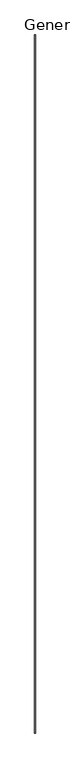
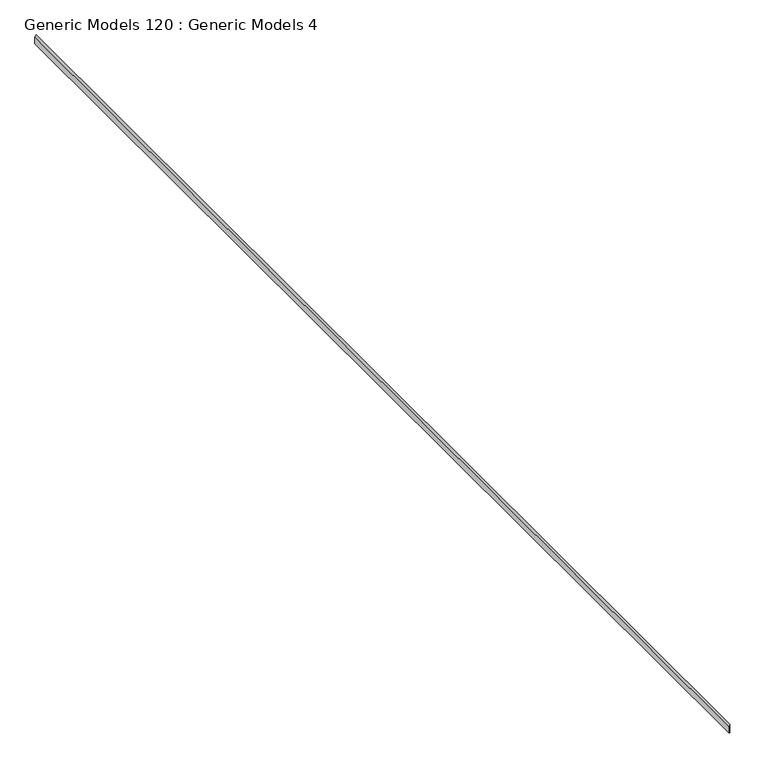
"""IFC4 building model written with IfcOpenShell, lengths in millimetres: proxy geometry, Generic Models 120 : Generic Models 4."""

from ifc_helpers import new_model, si_unit, frame, origin, place, context, project, spatial, polyline, outline, extrude, source, transform, mapped, element, save


def generic_models_120_generic_models_4_1dfd7883(model_context):
    return source(origin(), model_context, "Body", "SweptSolid", [
        extrude(outline(polyline([(126968.835011, 7259.1463704), (126963.120011, 7276.9263704), (127105.8556439, 7276.9263704), (127071.2314334, 7259.1463704), (126968.835011, 7259.1463704)])), frame((0.0, -6864.9230338, 0.0), z_axis=(0.0, 1.0, 0.0), x_axis=(0.0, 0.0, 1.0)), (0.0, 0.0, 1.0), 18643.6),
    ])


if __name__ == "__main__":
    model = new_model("IFC4")
    model_context = context("Model", 3, world=origin())
    ifc_project = project(units=[si_unit("LENGTHUNIT", "METRE", prefix="MILLI")], contexts=[model_context])
    site = spatial("IfcSite", under=ifc_project)
    building = spatial("IfcBuilding", under=site)
    placement = place(None, origin())
    generic_models_120_generic_models_4_shape = generic_models_120_generic_models_4_1dfd7883(model_context)
    element("IfcBuildingElementProxy", 1, Name="Generic Models 120 : Generic Models 4", ObjectType="Generic Models 120 : Generic Models 4", at=placement, inside=building, context=model_context, shape_type="MappedRepresentation", body=[
        mapped(generic_models_120_generic_models_4_shape, transform((0.0, 0.0, 0.0), x_axis=(1.0, 0.0, 0.0), y_axis=(0.0, 1.0, 0.0), z_axis=(0.0, 0.0, 1.0))),
    ])
    save(model, "model.ifc")

# Revit data of these elements
# Element 1 (IfcBuildingElementProxy, "Generic Models 120 : Generic Models 4")
#   Materials on its faces: "_7/8\" SMOOTH TROWEL EXTERIOR STUCCO (COLOR PER OWNER)"
# Materials
#   "_7/8\" SMOOTH TROWEL EXTERIOR STUCCO (COLOR PER OWNER)": class "Generic", colour RGB 233 233 233, transparency 0, Cost = 0
